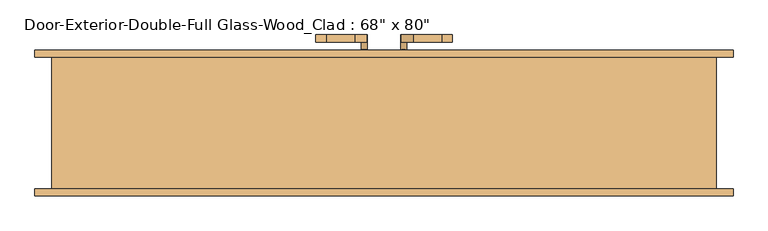
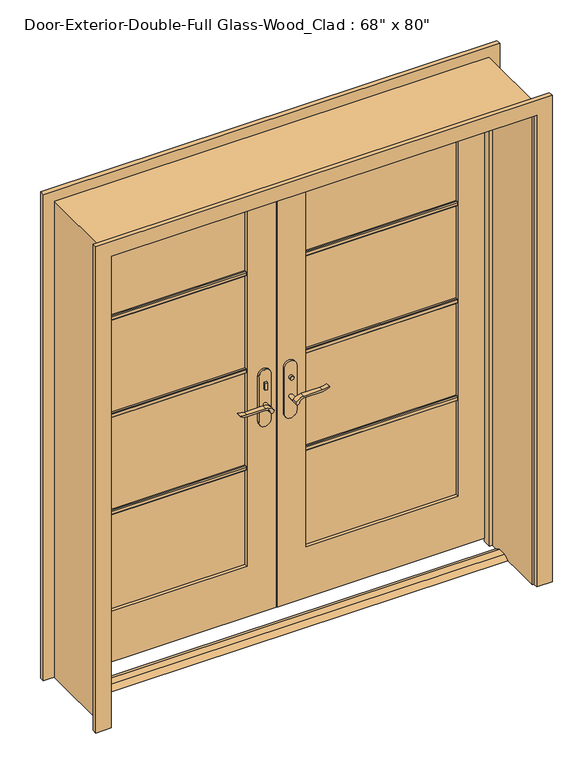
"""IFC4 building model written with IfcOpenShell, lengths in millimetres: door geometry."""

from ifc_helpers import new_model, si_unit, point, frame, frame_2d, origin, place, context, project, spatial, polyline, circle_curve, trimmed, segment, composite_curve, outline, extrude, faceted_brep, source, transform, mapped, element, save


def door_e0419d21(model_context):
    return source(origin(), model_context, "Body", "SolidModel", [
        extrude(outline(polyline([(19.05, 12.7), (53.975, 12.7), (79.375, 0.0), (-6.35, 0.0), (19.05, 12.7)])), frame((-863.6, 0.0, 0.0), z_axis=(1.0, 0.0, 0.0), x_axis=(0.0, 1.0, 0.0)), (0.0, 0.0, 1.0), 1727.2),
        extrude(outline(polyline([(-47.4019111, 118.1125), (-57.4019111, 118.1125), (-57.4019111, 128.1125), (-47.4019111, 128.1125), (-47.4019111, 118.1125)])), frame((0.0, 0.0, 981.9), z_axis=(0.0, 0.0, 1.0), x_axis=(1.0, 0.0, 0.0)), (0.0, 0.0, 1.0), 30.0),
        extrude(outline(composite_curve([segment(trimmed(circle_curve(frame_2d((996.9, -52.4019111)), 8.0), [point((996.9, -60.4019111))], [point((996.9, -44.4019111))], False, "CARTESIAN"), True, "CONTINUOUS"), segment(trimmed(circle_curve(frame_2d((996.9, -52.4019111)), 8.0), [point((996.9, -44.4019111))], [point((996.9, -60.4019111))], False, "CARTESIAN"), True, "CONTINUOUS")], self_intersect=False)), frame((0.0, 183.0375, 0.0), z_axis=(0.0, 1.0, 0.0), x_axis=(0.0, 0.0, 1.0)), (0.0, 0.0, 1.0), 10.0),
        extrude(outline(composite_curve([segment(trimmed(circle_curve(frame_2d((897.1555521, -76.0694241)), 37.2832219), [point((919.0523287, -45.8937749))], [point((934.4, -77.7693445))], False, "CARTESIAN"), True, "CONTINUOUS"), segment(polyline([(934.4, -77.7693445), (934.4, -154.045502)]), True, "CONTINUOUS"), segment(trimmed(circle_curve(frame_2d((1017.6850638, -153.9791202)), 83.2850902), [point((934.4, -154.045502))], [point((939.4, -182.4019111))], True, "CARTESIAN"), True, "CONTINUOUS"), segment(polyline([(939.4, -182.4019111), (936.6135558, -182.4019111)]), True, "CONTINUOUS"), segment(trimmed(circle_curve(frame_2d((986.6709207, -150.4622499)), 59.3791355), [point((936.6135558, -182.4019111))], [point((927.4, -154.045502))], False, "CARTESIAN"), True, "CONTINUOUS"), segment(polyline([(927.4, -154.045502), (927.4, -77.7881013)]), True, "CONTINUOUS"), segment(trimmed(circle_curve(frame_2d((909.2738613, -77.7881013)), 18.1261387), [point((927.4, -77.7881013))], [point((914.4, -60.4019111))], True, "CARTESIAN"), True, "CONTINUOUS"), segment(trimmed(circle_curve(frame_2d((914.4, -52.4019111)), 8.0), [point((914.4, -60.4019111))], [point((919.0523287, -45.8937749))], False, "CARTESIAN"), True, "CONTINUOUS")], self_intersect=False)), frame((0.0, 78.1125, 0.0), z_axis=(0.0, 1.0, 0.0), x_axis=(0.0, 0.0, 1.0)), (0.0, 0.0, 1.0), 20.0),
        extrude(outline(composite_curve([segment(trimmed(circle_curve(frame_2d((914.4, -52.4019111)), 8.0), [point((914.3999903, -60.4019111))], [point((919.0523287, -45.8937749))], False, "CARTESIAN"), True, "CONTINUOUS"), segment(trimmed(circle_curve(frame_2d((897.1555521, -76.0694241)), 37.2832219), [point((919.0523287, -45.8937749))], [point((934.4, -77.7693445))], False, "CARTESIAN"), True, "CONTINUOUS"), segment(polyline([(934.4, -77.7693445), (934.4, -154.045502)]), True, "CONTINUOUS"), segment(trimmed(circle_curve(frame_2d((1017.6850638, -153.9791202)), 83.2850902), [point((934.4, -154.045502))], [point((939.4, -182.4019111))], True, "CARTESIAN"), True, "CONTINUOUS"), segment(polyline([(939.4, -182.4019111), (936.6135558, -182.4019111)]), True, "CONTINUOUS"), segment(trimmed(circle_curve(frame_2d((986.6709207, -150.4622499)), 59.3791355), [point((936.6135558, -182.4019111))], [point((927.4, -154.045502))], False, "CARTESIAN"), True, "CONTINUOUS"), segment(polyline([(927.4, -154.045502), (927.4, -77.788099)]), True, "CONTINUOUS"), segment(trimmed(circle_curve(frame_2d((909.2738682, -77.788099)), 18.1261318), [point((927.4, -77.788099))], [point((914.3999903, -60.4019111))], True, "CARTESIAN"), True, "CONTINUOUS")], self_intersect=False)), frame((0.0, 213.0375, 0.0), z_axis=(0.0, 1.0, 0.0), x_axis=(0.0, 0.0, 1.0)), (0.0, 0.0, 1.0), 20.0),
        extrude(outline(composite_curve([segment(trimmed(circle_curve(frame_2d((914.4, -52.4019111)), 8.0), [point((914.4, -60.4019111))], [point((914.4, -44.4019111))], False, "CARTESIAN"), True, "CONTINUOUS"), segment(trimmed(circle_curve(frame_2d((914.4, -52.4019111)), 8.0), [point((914.4, -44.4019111))], [point((914.4, -60.4019111))], False, "CARTESIAN"), True, "CONTINUOUS")], self_intersect=False)), frame((0.0, 98.1125, 0.0), z_axis=(0.0, 1.0, 0.0), x_axis=(0.0, 0.0, 1.0)), (0.0, 0.0, 1.0), 30.0),
        extrude(outline(composite_curve([segment(trimmed(circle_curve(frame_2d((914.4, -52.4019111)), 8.0), [point((914.4, -60.4019111))], [point((914.4, -44.4019111))], False, "CARTESIAN"), True, "CONTINUOUS"), segment(trimmed(circle_curve(frame_2d((914.4, -52.4019111)), 8.0), [point((914.4, -44.4019111))], [point((914.4, -60.4019111))], False, "CARTESIAN"), True, "CONTINUOUS")], self_intersect=False)), frame((0.0, 183.0375, 0.0), z_axis=(0.0, 1.0, 0.0), x_axis=(0.0, 0.0, 1.0)), (0.0, 0.0, 1.0), 30.0),
        extrude(outline(composite_curve([segment(polyline([(844.4, -27.4019111), (1039.4, -27.4019111)]), True, "CONTINUOUS"), segment(trimmed(circle_curve(frame_2d((1039.4, -52.4019111)), 25.0), [point((1039.4, -27.4019111))], [point((1039.4, -77.4019111))], False, "CARTESIAN"), True, "CONTINUOUS"), segment(polyline([(1039.4, -77.4019111), (844.4, -77.4019111)]), True, "CONTINUOUS"), segment(trimmed(circle_curve(frame_2d((844.4, -52.4019111)), 25.0), [point((844.4, -77.4019111))], [point((844.4, -27.4019111))], False, "CARTESIAN"), True, "CONTINUOUS")], self_intersect=False)), frame((0.0, 128.1125, 0.0), z_axis=(0.0, 1.0, 0.0), x_axis=(0.0, 0.0, 1.0)), (0.0, 0.0, 1.0), 10.0),
        extrude(outline(composite_curve([segment(polyline([(844.4, -27.4019111), (1039.4, -27.4019111)]), True, "CONTINUOUS"), segment(trimmed(circle_curve(frame_2d((1039.4, -52.4019111)), 25.0), [point((1039.4, -27.4019111))], [point((1039.4, -77.4019111))], False, "CARTESIAN"), True, "CONTINUOUS"), segment(polyline([(1039.4, -77.4019111), (844.4, -77.4019111)]), True, "CONTINUOUS"), segment(trimmed(circle_curve(frame_2d((844.4, -52.4019111)), 25.0), [point((844.4, -77.4019111))], [point((844.4, -27.4019111))], False, "CARTESIAN"), True, "CONTINUOUS")], self_intersect=False)), frame((0.0, 173.0375, 0.0), z_axis=(0.0, 1.0, 0.0), x_axis=(0.0, 0.0, 1.0)), (0.0, 0.0, 1.0), 10.0),
        extrude(outline(polyline([(47.3875, 193.0375), (57.3875, 193.0375), (57.3875, 183.0375), (47.3875, 183.0375), (47.3875, 193.0375)])), frame((0.0, 0.0, 981.9), z_axis=(0.0, 0.0, 1.0), x_axis=(1.0, 0.0, 0.0)), (0.0, 0.0, 1.0), 30.0),
        extrude(outline(composite_curve([segment(trimmed(circle_curve(frame_2d((996.9, 52.3875)), 8.0), [point((996.9, 60.3875))], [point((996.9, 44.3875))], False, "CARTESIAN"), True, "CONTINUOUS"), segment(trimmed(circle_curve(frame_2d((996.9, 52.3875)), 8.0), [point((996.9, 44.3875))], [point((996.9, 60.3875))], False, "CARTESIAN"), True, "CONTINUOUS")], self_intersect=False)), frame((0.0, 118.1125, 0.0), z_axis=(0.0, 1.0, 0.0), x_axis=(0.0, 0.0, 1.0)), (0.0, 0.0, 1.0), 10.0),
        extrude(outline(composite_curve([segment(trimmed(circle_curve(frame_2d((914.4, 52.3875)), 8.0), [point((919.0523287, 45.8793637))], [point((914.4, 60.3875))], False, "CARTESIAN"), True, "CONTINUOUS"), segment(trimmed(circle_curve(frame_2d((909.2738613, 77.7736901)), 18.1261387), [point((914.4, 60.3875))], [point((927.4, 77.7736901))], True, "CARTESIAN"), True, "CONTINUOUS"), segment(polyline([(927.4, 77.7736901), (927.4, 154.0310909)]), True, "CONTINUOUS"), segment(trimmed(circle_curve(frame_2d((986.6709207, 150.4478388)), 59.3791355), [point((927.4, 154.0310909))], [point((936.6135558, 182.3875))], False, "CARTESIAN"), True, "CONTINUOUS"), segment(polyline([(936.6135558, 182.3875), (939.4, 182.3875)]), True, "CONTINUOUS"), segment(trimmed(circle_curve(frame_2d((1017.6850638, 153.9647091)), 83.2850902), [point((939.4, 182.3875))], [point((934.4, 154.0310909))], True, "CARTESIAN"), True, "CONTINUOUS"), segment(polyline([(934.4, 154.0310909), (934.4, 77.7549333)]), True, "CONTINUOUS"), segment(trimmed(circle_curve(frame_2d((897.1555521, 76.0550129)), 37.2832219), [point((934.4, 77.7549333))], [point((919.0523287, 45.8793637))], False, "CARTESIAN"), True, "CONTINUOUS")], self_intersect=False)), frame((0.0, 213.0375, 0.0), z_axis=(0.0, 1.0, 0.0), x_axis=(0.0, 0.0, 1.0)), (0.0, 0.0, 1.0), 20.0),
        extrude(outline(composite_curve([segment(trimmed(circle_curve(frame_2d((909.2738682, 77.7736878)), 18.1261318), [point((914.3999903, 60.3875))], [point((927.4, 77.7736878))], True, "CARTESIAN"), True, "CONTINUOUS"), segment(polyline([(927.4, 77.7736878), (927.4, 154.0310909)]), True, "CONTINUOUS"), segment(trimmed(circle_curve(frame_2d((986.6709207, 150.4478388)), 59.3791355), [point((927.4, 154.0310909))], [point((936.6135558, 182.3875))], False, "CARTESIAN"), True, "CONTINUOUS"), segment(polyline([(936.6135558, 182.3875), (939.4, 182.3875)]), True, "CONTINUOUS"), segment(trimmed(circle_curve(frame_2d((1017.6850638, 153.9647091)), 83.2850902), [point((939.4, 182.3875))], [point((934.4, 154.0310909))], True, "CARTESIAN"), True, "CONTINUOUS"), segment(polyline([(934.4, 154.0310909), (934.4, 77.7549333)]), True, "CONTINUOUS"), segment(trimmed(circle_curve(frame_2d((897.1555521, 76.0550129)), 37.2832219), [point((934.4, 77.7549333))], [point((919.0523287, 45.8793637))], False, "CARTESIAN"), True, "CONTINUOUS"), segment(trimmed(circle_curve(frame_2d((914.4, 52.3875)), 8.0), [point((919.0523287, 45.8793637))], [point((914.3999903, 60.3875))], False, "CARTESIAN"), True, "CONTINUOUS")], self_intersect=False)), frame((0.0, 78.1125, 0.0), z_axis=(0.0, 1.0, 0.0), x_axis=(0.0, 0.0, 1.0)), (0.0, 0.0, 1.0), 20.0),
        extrude(outline(composite_curve([segment(trimmed(circle_curve(frame_2d((914.4, 52.3875)), 8.0), [point((914.4, 60.3875))], [point((914.4, 44.3875))], False, "CARTESIAN"), True, "CONTINUOUS"), segment(trimmed(circle_curve(frame_2d((914.4, 52.3875)), 8.0), [point((914.4, 44.3875))], [point((914.4, 60.3875))], False, "CARTESIAN"), True, "CONTINUOUS")], self_intersect=False)), frame((0.0, 183.0375, 0.0), z_axis=(0.0, 1.0, 0.0), x_axis=(0.0, 0.0, 1.0)), (0.0, 0.0, 1.0), 30.0),
        extrude(outline(composite_curve([segment(trimmed(circle_curve(frame_2d((914.4, 52.3875)), 8.0), [point((914.4, 60.3875))], [point((914.4, 44.3875))], False, "CARTESIAN"), True, "CONTINUOUS"), segment(trimmed(circle_curve(frame_2d((914.4, 52.3875)), 8.0), [point((914.4, 44.3875))], [point((914.4, 60.3875))], False, "CARTESIAN"), True, "CONTINUOUS")], self_intersect=False)), frame((0.0, 98.1125, 0.0), z_axis=(0.0, 1.0, 0.0), x_axis=(0.0, 0.0, 1.0)), (0.0, 0.0, 1.0), 30.0),
        extrude(outline(composite_curve([segment(trimmed(circle_curve(frame_2d((844.4, 52.3875)), 25.0), [point((844.4, 27.3875))], [point((844.4, 77.3875))], False, "CARTESIAN"), True, "CONTINUOUS"), segment(polyline([(844.4, 77.3875), (1039.4, 77.3875)]), True, "CONTINUOUS"), segment(trimmed(circle_curve(frame_2d((1039.4, 52.3875)), 25.0), [point((1039.4, 77.3875))], [point((1039.4, 27.3875))], False, "CARTESIAN"), True, "CONTINUOUS"), segment(polyline([(1039.4, 27.3875), (844.4, 27.3875)]), True, "CONTINUOUS")], self_intersect=False)), frame((0.0, 173.0375, 0.0), z_axis=(0.0, 1.0, 0.0), x_axis=(0.0, 0.0, 1.0)), (0.0, 0.0, 1.0), 10.0),
        extrude(outline(composite_curve([segment(trimmed(circle_curve(frame_2d((844.4, 52.3875)), 25.0), [point((844.4, 27.3875))], [point((844.4, 77.3875))], False, "CARTESIAN"), True, "CONTINUOUS"), segment(polyline([(844.4, 77.3875), (1039.4, 77.3875)]), True, "CONTINUOUS"), segment(trimmed(circle_curve(frame_2d((1039.4, 52.3875)), 25.0), [point((1039.4, 77.3875))], [point((1039.4, 27.3875))], False, "CARTESIAN"), True, "CONTINUOUS"), segment(polyline([(1039.4, 27.3875), (844.4, 27.3875)]), True, "CONTINUOUS")], self_intersect=False)), frame((0.0, 128.1125, 0.0), z_axis=(0.0, 1.0, 0.0), x_axis=(0.0, 0.0, 1.0)), (0.0, 0.0, 1.0), 10.0),
        extrude(outline(polyline([(152.0825, 1502.171875), (152.0825, 1483.121875), (145.7325, 1483.121875), (142.5575, 1486.296875), (142.5575, 1498.996875), (145.7325, 1502.171875), (152.0825, 1502.171875)])), frame((120.65, 0.0, 0.0), z_axis=(1.0, 0.0, 0.0), x_axis=(0.0, 1.0, 0.0)), (0.0, 0.0, 1.0), 622.3),
        extrude(outline(polyline([(152.0825, 1081.88125), (152.0825, 1062.83125), (145.7325, 1062.83125), (142.5575, 1066.00625), (142.5575, 1078.70625), (145.7325, 1081.88125), (152.0825, 1081.88125)])), frame((120.65, 0.0, 0.0), z_axis=(1.0, 0.0, 0.0), x_axis=(0.0, 1.0, 0.0)), (0.0, 0.0, 1.0), 622.3),
        extrude(outline(polyline([(152.0825, 661.590625), (152.0825, 642.540625), (145.7325, 642.540625), (142.5575, 645.715625), (142.5575, 658.415625), (145.7325, 661.590625), (152.0825, 661.590625)])), frame((120.65, 0.0, 0.0), z_axis=(1.0, 0.0, 0.0), x_axis=(0.0, 1.0, 0.0)), (0.0, 0.0, 1.0), 622.3),
        extrude(outline(polyline([(159.0675, 1502.171875), (165.4175, 1502.171875), (168.5925, 1498.996875), (168.5925, 1486.296875), (165.4175, 1483.121875), (159.0675, 1483.121875), (159.0675, 1502.171875)])), frame((-742.95, 0.0, 0.0), z_axis=(1.0, 0.0, 0.0), x_axis=(0.0, 1.0, 0.0)), (0.0, 0.0, 1.0), 622.3),
        extrude(outline(polyline([(159.0675, 1081.88125), (165.4175, 1081.88125), (168.5925, 1078.70625), (168.5925, 1066.00625), (165.4175, 1062.83125), (159.0675, 1062.83125), (159.0675, 1081.88125)])), frame((-742.95, 0.0, 0.0), z_axis=(1.0, 0.0, 0.0), x_axis=(0.0, 1.0, 0.0)), (0.0, 0.0, 1.0), 622.3),
        extrude(outline(polyline([(159.0675, 661.590625), (165.4175, 661.590625), (168.5925, 658.415625), (168.5925, 645.715625), (165.4175, 642.540625), (159.0675, 642.540625), (159.0675, 661.590625)])), frame((-742.95, 0.0, 0.0), z_axis=(1.0, 0.0, 0.0), x_axis=(0.0, 1.0, 0.0)), (0.0, 0.0, 1.0), 622.3),
        extrude(outline(polyline([(159.0675, 1502.171875), (165.4175, 1502.171875), (168.5925, 1498.996875), (168.5925, 1486.296875), (165.4175, 1483.121875), (159.0675, 1483.121875), (159.0675, 1502.171875)])), frame((120.65, 0.0, 0.0), z_axis=(1.0, 0.0, 0.0), x_axis=(0.0, 1.0, 0.0)), (0.0, 0.0, 1.0), 622.3),
        extrude(outline(polyline([(159.0675, 1081.88125), (165.4175, 1081.88125), (168.5925, 1078.70625), (168.5925, 1066.00625), (165.4175, 1062.83125), (159.0675, 1062.83125), (159.0675, 1081.88125)])), frame((120.65, 0.0, 0.0), z_axis=(1.0, 0.0, 0.0), x_axis=(0.0, 1.0, 0.0)), (0.0, 0.0, 1.0), 622.3),
        extrude(outline(polyline([(159.0675, 661.590625), (165.4175, 661.590625), (168.5925, 658.415625), (168.5925, 645.715625), (165.4175, 642.540625), (159.0675, 642.540625), (159.0675, 661.590625)])), frame((120.65, 0.0, 0.0), z_axis=(1.0, 0.0, 0.0), x_axis=(0.0, 1.0, 0.0)), (0.0, 0.0, 1.0), 622.3),
        extrude(outline(polyline([(152.0825, 1502.171875), (152.0825, 1483.121875), (145.7325, 1483.121875), (142.5575, 1486.296875), (142.5575, 1498.996875), (145.7325, 1502.171875), (152.0825, 1502.171875)])), frame((-742.95, 0.0, 0.0), z_axis=(1.0, 0.0, 0.0), x_axis=(0.0, 1.0, 0.0)), (0.0, 0.0, 1.0), 622.3),
        extrude(outline(polyline([(152.0825, 1081.88125), (152.0825, 1062.83125), (145.7325, 1062.83125), (142.5575, 1066.00625), (142.5575, 1078.70625), (145.7325, 1081.88125), (152.0825, 1081.88125)])), frame((-742.95, 0.0, 0.0), z_axis=(1.0, 0.0, 0.0), x_axis=(0.0, 1.0, 0.0)), (0.0, 0.0, 1.0), 622.3),
        extrude(outline(polyline([(152.0825, 661.590625), (152.0825, 642.540625), (145.7325, 642.540625), (142.5575, 645.715625), (142.5575, 658.415625), (145.7325, 661.590625), (152.0825, 661.590625)])), frame((-742.95, 0.0, 0.0), z_axis=(1.0, 0.0, 0.0), x_axis=(0.0, 1.0, 0.0)), (0.0, 0.0, 1.0), 622.3),
        extrude(outline(polyline([(0.0, 869.95), (0.0, 933.45), (2101.85, 933.45), (2101.85, -933.45), (0.0, -933.45), (0.0, -869.95), (2038.35, -869.95), (2038.35, 869.95), (0.0, 869.95)])), frame((0.0, 173.0375, 0.0), z_axis=(0.0, 1.0, 0.0), x_axis=(0.0, 0.0, 1.0)), (0.0, 0.0, 1.0), 19.05),
        extrude(outline(polyline([(0.0, 869.95), (0.0, 933.45), (2101.85, 933.45), (2101.85, -933.45), (0.0, -933.45), (0.0, -869.95), (2038.35, -869.95), (2038.35, 869.95), (0.0, 869.95)])), frame((0.0, -198.4375, 0.0), z_axis=(0.0, 1.0, 0.0), x_axis=(0.0, 0.0, 1.0)), (0.0, 0.0, 1.0), 19.05),
        extrude(outline(polyline([(12.7, 863.6), (2032.0, 863.6), (2032.0, 1.5875), (12.7, 1.5875), (12.7, 863.6)]), holes=[polyline([(1912.9375, 120.65), (1912.9375, 742.95), (231.775, 742.95), (231.775, 120.65), (1912.9375, 120.65)])]), frame((0.0, 138.1125, 0.0), z_axis=(0.0, 1.0, 0.0), x_axis=(0.0, 0.0, 1.0)), (0.0, 0.0, 1.0), 34.925),
        extrude(outline(polyline([(2032.0, -863.6), (12.7, -863.6), (12.7, -1.6019111), (2032.0, -1.6019111), (2032.0, -863.6)]), holes=[polyline([(231.775, -742.95), (1912.9375, -742.95), (1912.9375, -120.65), (231.775, -120.65), (231.775, -742.95)])]), frame((0.0, 138.1125, 0.0), z_axis=(0.0, 1.0, 0.0), x_axis=(0.0, 0.0, 1.0)), (0.0, 0.0, 1.0), 34.925),
        faceted_brep([(889.0, 173.0375, 0.0), (889.0, -179.3875, 0.0), (863.6, -179.3875, 0.0), (863.6, 103.1875, 0.0), (850.9, 103.1875, 0.0), (850.9, 138.1125, 0.0), (863.6, 138.1125, 0.0), (863.6, 173.0375, 0.0), (889.0, 173.0375, 2057.4), (889.0, -179.3875, 2057.4), (-889.0, -179.3875, 2057.4), (-889.0, -179.3875, 0.0), (-863.6, -179.3875, 0.0), (-863.6, -179.3875, 2032.0), (863.6, -179.3875, 2032.0), (863.6, 103.1875, 2032.0), (-863.6, 103.1875, 2032.0), (-863.6, 103.1875, 0.0), (-850.9, 103.1875, 0.0), (-850.9, 103.1875, 2019.3), (850.9, 103.1875, 2019.3), (850.9, 138.1125, 2019.3), (1.5875, 138.1125, 2019.3), (-1.6019111, 138.1125, 2019.3), (-850.9, 138.1125, 2019.3), (-850.9, 138.1125, 0.0), (-863.6, 138.1125, 0.0), (-863.6, 138.1125, 2032.0), (-1.6019111, 138.1125, 2032.0), (1.5875, 138.1125, 2032.0), (863.6, 138.1125, 2032.0), (863.6, 173.0375, 2032.0), (1.5875, 173.0375, 2032.0), (-1.6019111, 173.0375, 2032.0), (-863.6, 173.0375, 2032.0), (-863.6, 173.0375, 0.0), (-889.0, 173.0375, 0.0), (-889.0, 173.0375, 2057.4)], [[[0, 1, 2, 3, 4, 5, 6, 7]], [[1, 0, 8, 9]], [[2, 1, 9, 10, 11, 12, 13, 14]], [[3, 2, 14, 15]], [[4, 3, 15, 16, 17, 18, 19, 20]], [[5, 4, 20, 21]], [[6, 5, 21, 22, 23, 24, 25, 26, 27, 28, 29, 30]], [[7, 6, 30, 31]], [[0, 7, 31, 32, 33, 34, 35, 36, 37, 8]], [[9, 8, 37, 10]], [[14, 13, 16, 15]], [[20, 19, 24, 23, 22, 21]], [[31, 30, 29, 28, 27, 34, 33, 32]], [[12, 11, 36, 35, 26, 25, 18, 17]], [[11, 10, 37, 36]], [[13, 12, 17, 16]], [[19, 18, 25, 24]], [[27, 26, 35, 34]]]),
        extrude(outline(polyline([(742.95, 152.0825), (120.65, 152.0825), (120.65, 159.0675), (742.95, 159.0675), (742.95, 152.0825)])), frame((0.0, 0.0, 231.775), z_axis=(0.0, 0.0, 1.0), x_axis=(1.0, 0.0, 0.0)), (0.0, 0.0, 1.0), 1681.1625),
        extrude(outline(polyline([(-120.65, 152.0825), (-742.95, 152.0825), (-742.95, 159.0675), (-120.65, 159.0675), (-120.65, 152.0825)])), frame((0.0, 0.0, 231.775), z_axis=(0.0, 0.0, 1.0), x_axis=(1.0, 0.0, 0.0)), (0.0, 0.0, 1.0), 1681.1625),
    ])


if __name__ == "__main__":
    model = new_model("IFC4")
    model_context = context("Model", 3, world=origin())
    ifc_project = project(units=[si_unit("LENGTHUNIT", "METRE", prefix="MILLI")], contexts=[model_context])
    site = spatial("IfcSite", under=ifc_project)
    building = spatial("IfcBuilding", under=site)
    placement = place(None, origin())
    door_shape = door_e0419d21(model_context)
    element("IfcDoor", 1, ObjectType="Door-Exterior-Double-Full Glass-Wood_Clad : 68\" x 80\"", at=placement, inside=building, context=model_context, shape_type="MappedRepresentation", body=[
        mapped(door_shape, transform((0.0, 0.0, 0.0), x_axis=(1.0, 0.0, 0.0), y_axis=(0.0, 1.0, 0.0), z_axis=(0.0, 0.0, 1.0))),
    ])
    save(model, "model.ifc")

# Revit data of these elements
# Type "Door-Exterior-Double-Full Glass-Wood_Clad : 68\" x 80\""
#   Type Mark = "21"
#   Assembly Code = "B2030100"
#   Analytic Construction = "French door, wood frame with double glass"
#   Top Rail = 0' - 4 11/16"
#   Threshold Offset [instance default] = 0' - 0 1/2"
#   Thickness = 0' - 1 3/8"
#   Thermal Resistance (R) = 1.9158 (h·ft²·°F)/BTU
#   Swing Angle [instance default] = 90.0000°
#   Stiles = 0' - 4 3/4"
#   Rough Width = 5' - 10"
#   Rough Height = 6' - 9"
#   Panel Width = 2' - 10"
#   Door Offset [instance default] = 0' - 0"
#   Height = 6' - 8"
#   Width = 5' - 8"
#   Heat Transfer Coefficient (U) = 0.5220 BTU/(h·ft²·°F)
#   Bottom Rail = 0' - 9 1/8"
#   Exterior Trim [instance default] = yes
#   Threshold [instance default] = yes
#   Show Grill [instance default] = yes
#   Function = 1
#   Trim Material = Cherry
#   Threshold Material = Cherry
#   Panel Material = Cherry
#   Glazing = Glass
#   Frame Material = Cherry
#   Door Handle Material = Aluminum
#   Visual Light Transmittance = 0
#   Solar Heat Gain Coefficient = 0
#   Wall Closure = (empty or 0)
#   Construction Type = (empty or 0)
# Element 1 (IfcDoor, "Door-Exterior-Double-Full Glass-Wood_Clad : 68\" x 80\"")
#   Materials on its faces: "Cherry", "Aluminum", "Glass"
# Materials
#   "Cherry": class "Wood", colour RGB 226 177 128, transparency 0, Description = "Prunus Serotina", Cost = 0
#   "Glass": class "Glass", colour RGB 0 128 192, transparency 0.75, Description = "Soda Lime Glass", Cost = 0
#   "Aluminum": class "Metal", colour RGB 247 247 247, transparency 0, Description = "Aluminum 6061", Cost = 0
